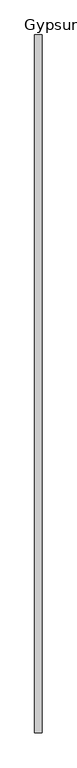
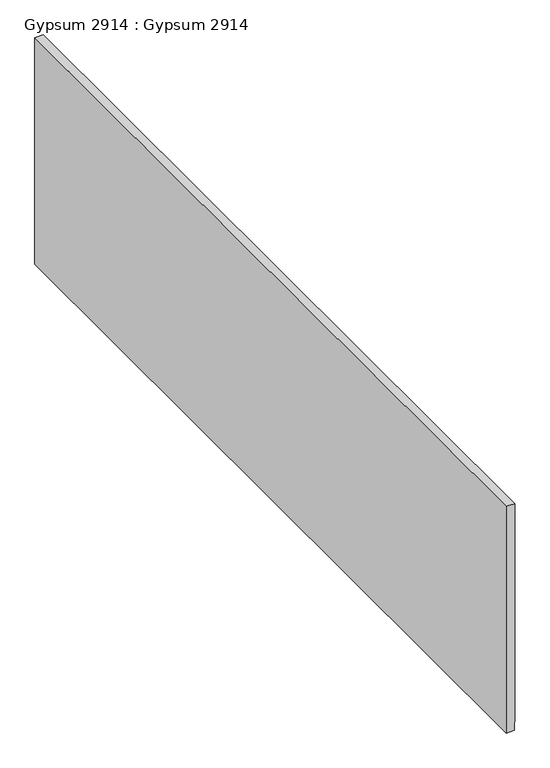
"""IFC4 building model written with IfcOpenShell, lengths in millimetres: proxy geometry, Gypsum 2914 : Gypsum 2914."""

from ifc_helpers import new_model, si_unit, frame, origin, place, context, project, spatial, polyline, outline, extrude, source, transform, mapped, element, save


def gypsum_2914_gypsum_2914_eb470674(model_context):
    return source(origin(), model_context, "Body", "SweptSolid", [
        extrude(outline(polyline([(39545.1675708, -640.491476), (39567.6883323, -640.491476), (39567.6883323, -639.211476), (40131.746, -639.211476), (40131.746, -660.156476), (39545.1675708, -660.156476), (39545.1675708, -640.491476)])), frame((0.0, -1052.8906574, 0.0), z_axis=(0.0, 1.0, 0.0), x_axis=(0.0, 0.0, 1.0)), (0.0, 0.0, 1.0), 2000.0),
    ])


if __name__ == "__main__":
    model = new_model("IFC4")
    model_context = context("Model", 3, world=origin())
    ifc_project = project(units=[si_unit("LENGTHUNIT", "METRE", prefix="MILLI")], contexts=[model_context])
    site = spatial("IfcSite", under=ifc_project)
    building = spatial("IfcBuilding", under=site)
    placement = place(None, origin())
    gypsum_2914_gypsum_2914_shape = gypsum_2914_gypsum_2914_eb470674(model_context)
    element("IfcBuildingElementProxy", 1, Name="Gypsum 2914 : Gypsum 2914", ObjectType="Gypsum 2914 : Gypsum 2914", at=placement, inside=building, context=model_context, shape_type="MappedRepresentation", body=[
        mapped(gypsum_2914_gypsum_2914_shape, transform((0.0, 0.0, 0.0), x_axis=(1.0, 0.0, 0.0), y_axis=(0.0, 1.0, 0.0), z_axis=(0.0, 0.0, 1.0))),
    ])
    save(model, "model.ifc")

# Revit data of these elements
# Type "Gypsum 2914 : Gypsum 2914"
#   NameOverride = "Gypsum"
# Element 1 (IfcBuildingElementProxy, "Gypsum 2914 : Gypsum 2914")
#   Materials on its faces: "5/8\" GYPSUM BOARD"
# Materials
#   "5/8\" GYPSUM BOARD": class "Unassigned", colour RGB 255 255 255, transparency 0, Cost = 0
